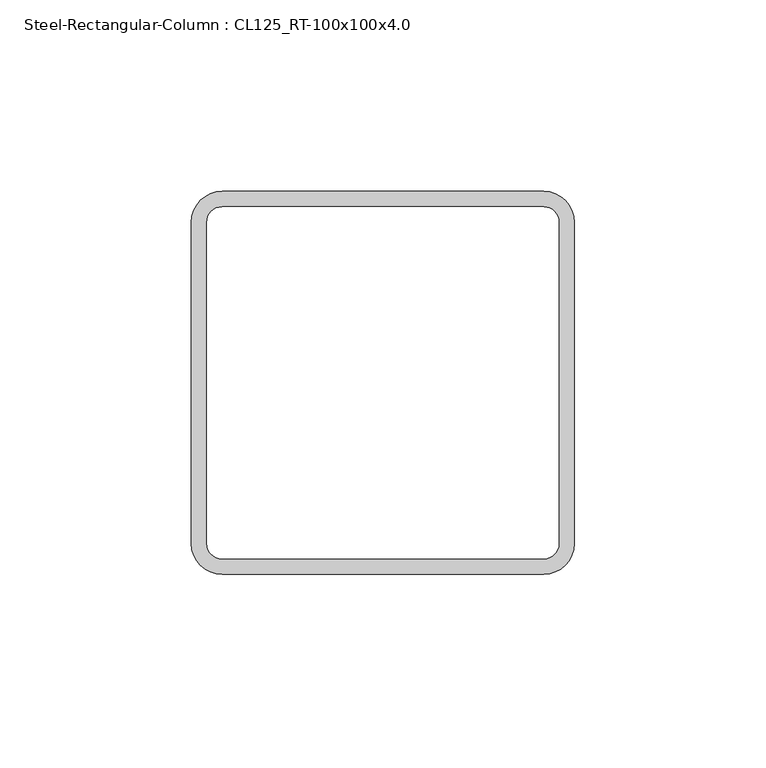
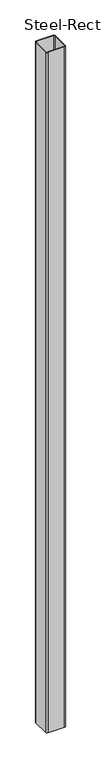
# IFC4 building model written with IfcOpenShell, lengths in millimetres: column geometry, Steel-Rectangular-Column : CL125_RT-100x100x4.0.
# Revit data of these elements (continued)
# Project information (continued)
#     -cfd758078946\" /><element revit_id=\"af7cfdda-f71a-4a09-bb03-63e0c16d5d93-001530cf\" ism_id=\"46a5ded9-4fed-43a0-a06e-bb0fce603002\" /><element revit_id=\"af7cfdda-f71a-4a09-bb03-63e0c16d5d93-001530d1\" ism_id=\"62d05a0c-55f2-4c29-a355-b77f91c84c50\" /><element revit_id=\"af7cfdda-f71a-4a09-bb03-63e0c16d5d93-001530d3\" ism_id=\"eac0c420-7041-45a3-ad98-0cab4f5d8155\" /><element revit_id=\"af7cfdda-f71a-4a09-bb03-63e0c16d5d93-001530d5\" ism_id=\"9f5beb51-429a-4c7b-aa2e-ad2efe601ed6\" /><element revit_id=\"af7cfdda-f71a-4a09-bb03-63e0c16d5d93-001530d7\" ism_id=\"4613af3e-a189-4781-a937-106d789655c9\" /><element revit_id=\"af7cfdda-f71a-4a09-bb03-63e0c16d5d93-001530d9\" ism_id=\"71402e21-51c1-43b7-b8cc-75d2aba247eb\" /><element revit_id=\"af7cfdda-f71a-4a09-bb03-63e0c16d5d93-001530db\" ism_id=\"89101b83-9b84-4f11-b026-90cd564a3900\" /><element revit_id=\"af7cfdda-f71a-4a09-bb03-63e0c16d5d93-001530dd\" ism_id=\"37670781-ce23-4ce1-992b-7a400613c37b\" /><element revit_id=\"af7cfdda-f71a-4a09-bb03-63e0c16d5d93-001530df\" ism_id=\"2316856d-18eb-466b-8ab8-114816378db0\" /><element revit_id=\"af7cfdda-f71a-4a09-bb03-63e0c16d5d93-001530e2\" ism_id=\"da4f1597-5b5a-43a6-aa94-e478ffd6cfc7\" /><element revit_id=\"af7cfdda-f71a-4a09-bb03-63e0c16d5d93-001530e5\" ism_id=\"60805764-efb2-4434-8d81-aed3c3ed3c1b\" /><element revit_id=\"af7cfdda-f71a-4a09-bb03-63e0c16d5d93-001530e8\" ism_id=\"34e34ebb-6481-4bfb-b3d0-cb52295ff652\" /><element revit_id=\"af7cfdda-f71a-4a09-bb03-63e0c16d5d93-001530eb\" ism_id=\"dd5c4d73-1406-4c40-a955-5f9c52d01161\" /><element revit_id=\"af7cfdda-f71a-4a09-bb03-63e0c16d5d93-001530ed\" ism_id=\"cf8abc6b-638f-4bd5-8b66-615be032e220\" /><element revit_id=\"af7cfdda-f71a-4a09-bb03-63e0c16d5d93-001530f0\" ism_id=\"56ce8857-0c24-48d5-82f2-459e263998e2\" /><element revit_id=\"af7cfdda-f71a-4a09-bb03-63e0c16d5d93-001530f2\" ism_id=\"a1f000e8-ea08-442b-8a96-da7657653fd5\" /><element revit_id=\"af7cfdda-f71a-4a09-bb03-63e0c16d5d93-001530f4\" ism_id=\"2625e954-f7fb-41eb-b9bd-1b615ef945fc\" /><element revit_id=\"af7cfdda-f71a-4a09-bb03-63e0c16d5d93-001530f6\" ism_id=\"48469362-393c-4deb-bbb2-ad00180a23fb\" /><element revit_id=\"af7cfdda-f71a-4a09-bb03-63e0c16d5d93-001530f8\" ism_id=\"8e650f6f-0906-45a9-8fb8-35680155d6db\" /><element revit_id=\"af7cfdda-f71a-4a09-bb03-63e0c16d5d93-001530fb\" ism_id=\"f84acaf6-20a1-4df6-afed-1dc07fd0b2e9\" /><element revit_id=\"af7cfdda-f71a-4a09-bb03-63e0c16d5d93-001530fe\" ism_id=\"72816c7e-9128-47f4-b46a-ee567a2a03d6\" /><element revit_id=\"af7cfdda-f71a-4a09-bb03-63e0c16d5d93-00153100\" ism_id=\"c95ab0f8-b4bf-4b7c-bd1d-0423c8ac725a\" /><element revit_id=\"af7cfdda-f71a-4a09-bb03-63e0c16d5d93-00153102\" ism_id=\"32fd4119-6673-4973-aef2-b39ef90310e5\" /><element revit_id=\"af7cfdda-f71a-4a09-bb03-63e0c16d5d93-00153104\" ism_id=\"fd2aa4a6-d123-4100-85b9-db27c20cf6bc\" /><element revit_id=\"af7cfdda-f71a-4a09-bb03-63e0c16d5d93-00153106\" ism_id=\"e00fdefa-e77c-4406-9dbe-3c9122259821\" /><element revit_id=\"af7cfdda-f71a-4a09-bb03-63e0c16d5d93-00153108\" ism_id=\"25e5b79e-07c2-4ffa-a7a9-bf039dd2ad78\" /><element revit_id=\"af7cfdda-f71a-4a09-bb03-63e0c16d5d93-0015310b\" ism_id=\"720021d4-ca74-47c0-9c64-7d0854fa39f5\" /><element revit_id=\"af7cfdda-f71a-4a09-bb03-63e0c16d5d93-0015310d\" ism_id=\"ea922120-0cff-4f8d-a5c2-2841c031873e\" /><element revit_id=\"af7cfdda-f71a-4a09-bb03-63e0c16d5d93-0015310f\" ism_id=\"9d07ca73-3a65-44fe-ab61-476d8d1352d1\" /><element revit_id=\"af7cfdda-f71a-4a09-bb03-63e0c16d5d93-00153111\" ism_id=\"68a2fb30-d213-40c7-a166-dad5a20bd269\" /><element revit_id=\"af7cfdda-f71a-4a09-bb03-63e0c16d5d93-00153113\" ism_id=\"06119775-28f9-44f0-a265-5c57029016d1\" /><element revit_id=\"af7cfdda-f71a-4a09-bb03-63e0c16d5d93-00153115\" ism_id=\"ca133383-8253-4d07-aa92-f507fbb2ee47\" /><element revit_id=\"af7cfdda-f71a-4a09-bb03-63e0c16d5d93-00153117\" ism_id=\"6f4a7c07-4bd3-4c99-b1e4-110c964ccc07\" /><element revit_id=\"af7cfdda-f71a-4a09-bb03-63e0c16d5d93-00153119\" ism_id=\"ee1f865b-98a9-4ff1-a84c-52926e8f3566\" /><element revit_id=\"af7cfdda-f71a-4a09-bb03-63e0c16d5d93-0015311b\" ism_id=\"4fd7bd5c-7c46-4e79-a72b-dab4a1d98f33\" /><element revit_id=\"af7cfdda-f71a-4a09-bb03-63e0c16d5d93-0015311e\" ism_id=\"9ca0cac6-aaff-412a-b9c1-a8be985bc44a\" /><element revit_id=\"af7cfdda-f71a-4a09-bb03-63e0c16d5d93-00153121\" ism_id=\"73123639-76b5-46f0-a49e-b26af36d93b1\" /><element revit_id=\"af7cfdda-f71a-4a09-bb03-63e0c16d5d93-00153123\" ism_id=\"f74e8cb9-a93d-4aaa-985b-c0ed9befad19\" /><element revit_id=\"af7cfdda-f71a-4a09-bb03-63e0c16d5d93-00153126\" ism_id=\"5778daa1-b4cb-4cc3-9b7d-323562a47fba\" /><element revit_id=\"af7cfdda-f71a-4a09-bb03-63e0c16d5d93-00153129\" ism_id=\"2d7457d2-8978-4c95-9056-ebbaed3263eb\" /><element revit_id=\"af7cfdda-f71a-4a09-bb03-63e0c16d5d93-0015312c\" ism_id=\"48b420ce-6767-430a-aadc-695c25361a2d\" /><element revit_id=\"af7cfdda-f71a-4a09-bb03-63e0c16d5d93-0015312e\" ism_id=\"fc34038c-136d-4d55-b951-9cc35899fd33\" /><element revit_id=\"af7cfdda-f71a-4a09-bb03-63e0c16d5d93-00153130\" ism_id=\"e7a25938-3b91-4519-a48d-86fdd79489d5\" /><element revit_id=\"af7cfdda-f71a-4a09-bb03-63e0c16d5d93-00153133\" ism_id=\"c81dfd8c-579c-4d77-ab89-bf1f415d9cc6\" /><element revit_id=\"af7cfdda-f71a-4a09-bb03-63e0c16d5d93-00153136\" ism_id=\"5756a4b4-84ca-418c-b9f6-2d2370afca2f\" /><element revit_id=\"af7cfdda-f71a-4a09-bb03-63e0c16d5d93-0015313a\" ism_id=\"09a9cede-a757-4d8e-a722-6140af98bc61\" /><element revit_id=\"af7cfdda-f71a-4a09-bb03-63e0c16d5d93-0015313d\" ism_id=\"ac9b583c-7f63-4351-8b69-3967279b234c\" /><element revit_id=\"af7cfdda-f71a-4a09-bb03-63e0c16d5d93-00153140\" ism_id=\"1a52584d-6b21-4de6-bb42-5b9bdd6f24e9\" /><element revit_id=\"af7cfdda-f71a-4a09-bb03-63e0c16d5d93-00153143\" ism_id=\"6c2e2bc0-8432-4c98-9292-cbb2182bd4b0\" /><element revit_id=\"af7cfdda-f71a-4a09-bb03-63e0c16d5d93-00153145\" ism_id=\"644bb900-7654-42c5-a9b7-996a2197f6d0\" /><element revit_id=\"af7cfdda-f71a-4a09-bb03-63e0c16d5d93-00153148\" ism_id=\"a1bca0bd-75db-464c-b27a-2a69d9b4ad3d\" /><element revit_id=\"af7cfdda-f71a-4a09-bb03-63e0c16d5d93-0015314a\" ism_id=\"ea29955b-34f2-409a-aefa-e6adfe75349e\" /><element revit_id=\"af7cfdda-f71a-4a09-bb03-63e0c16d5d93-0015314d\" ism_id=\"800fef33-e5e1-422c-b708-e9394bbeefcc\" /><element revit_id=\"af7cfdda-f71a-4a09-bb03-63e0c16d5d93-0015314f\" ism_id=\"86259dca-8773-4253-ac56-e71252267c8a\" /><element revit_id=\"af7cfdda-f71a-4a09-bb03-63e0c16d5d93-00153152\" ism_id=\"d15a0ad2-db9f-420d-bea3-41a78a0eb330\" /><element revit_id=\"af7cfdda-f71a-4a09-bb03-63e0c16d5d93-00153155\" ism_id=\"bd27f420-df49-4abe-bd96-8e48e7f4efcb\" /><element revit_id=\"af7cfdda-f71a-4a09-bb03-63e0c16d5d93-00153157\" ism_id=\"5d451f94-860d-4cc3-a4fa-51a9f3126e33\" /><element revit_id=\"af7cfdda-f71a-4a09-bb03-63e0c16d5d93-0015315a\" ism_id=\"4234158a-994a-492b-85da-6108709b7232\" /><element revit_id=\"af7cfdda-f71a-4a09-bb03-63e0c16d5d93-0015315c\" ism_id=\"ca24c92d-986b-417f-812f-024ab15e24c8\" /><element revit_id=\"af7cfdda-f71a-4a09-bb03-63e0c16d5d93-0015315f\" ism_id=\"699ec3b0-0151-4110-b054-14418651f324\" /><element revit_id=\"af7cfdda-f71a-4a09-bb03-63e0c16d5d93-00153161\" ism_id=\"38ecdeac-3d85-48dd-82c1-53fe93f49beb\" /><element revit_id=\"af7cfdda-f71a-4a09-bb03-63e0c16d5d93-00153163\" ism_id=\"1340aefd-b79c-4264-8a49-d0a0504eff8c\" /><element revit_id=\"af7cfdda-f71a-4a09-bb03-63e0c16d5d93-00153165\" ism_id=\"1b6167c2-fb26-4b8d-916b-d835d89896e7\" /><element revit_id=\"af7cfdda-f71a-4a09-bb03-63e0c16d5d93-00153167\" ism_id=\"290d3d83-57eb-4125-aecb-a977a5fcf5ca\" /><element revit_id=\"af7cfdda-f71a-4a09-bb03-63e0c16d5d93-00153169\" ism_id=\"105c9b97-1c70-4237-82ac-8404a3e8e6a6\" /><element revit_id=\"af7cfdda-f71a-4a09-bb03-63e0c16d5d93-0015316c\" ism_id=\"1726c5bb-05e2-4959-9da2-4227f0219f00\" /><element revit_id=\"af7cfdda-f71a-4a09-bb03-63e0c16d5d93-0015316e\" ism_id=\"d919ee9c-caed-4119-b451-e3644db952c8\" /><element revit_id=\"af7cfdda-f71a-4a09-bb03-63e0c16d5d93-00153170\" ism_id=\"1b1fab26-60c4-40ed-b31b-b177eda246ce\" /><element revit_id=\"af7cfdda-f71a-4a09-bb03-63e0c16d5d93-00153172\" ism_id=\"ea9b5221-a1f2-4796-8cca-f7872ab69cbd\" /><element revit_id=\"af7cfdda-f71a-4a09-bb03-63e0c16d5d93-00153174\" ism_id=\"660b40b2-06fb-4b62-b987-28a171e473fe\" /><element revit_id=\"af7cfdda-f71a-4a09-bb03-63e0c16d5d93-00153176\" ism_id=\"767be0d9-c5ba-4ad3-a52d-efd60031fc9a\" /><element revit_id=\"af7cfdda-f71a-4a09-bb03-63e0c16d5d93-00153178\" ism_id=\"6fbe93ce-4ed7-4596-88fc-71dafe48803e\" /><element revit_id=\"af7cfdda-f71a-4a09-bb03-63e0c16d5d93-0015317a\" ism_id=\"27d7b093-4eb7-47aa-b123-5388a6327d7f\" /><element revit_id=\"af7cfdda-f71a-4a09-bb03-63e0c16d5d93-0015317c\" ism_id=\"9073a947-5952-42fe-b37a-cdfed3ca30c7\" /><element revit_id=\"af7cfdda-f71a-4a09-bb03-63e0c16d5d93-0015317e\" ism_id=\"1888f060-aa3c-4494-8f30-a80ca2311216\" /><element revit_id=\"af7cfdda-f71a-4a09-bb03-63e0c16d5d93-00153181\" ism_id=\"c0491dc2-5df2-4c14-b988-e117f6f511a2\" /><element revit_id=\"af7cfdda-f71a-4a09-bb03-63e0c16d5d93-00153184\" ism_id=\"4f44b9aa-c092-46fe-bf9b-2d1be872d419\" /><element revit_id=\"af7cfdda-f71a-4a09-bb03-63e0c16d5d93-00153186\" ism_id=\"eb560801-76cf-40a8-a181-31cd32aca14f\" /><element revit_id=\"af7cfdda-f71a-4a09-bb03-63e0c16d5d93-00153189\" ism_id=\"8d1e5f00-41d5-42c1-9b4f-a8c2eb689a72\" /><element revit_id=\"af7cfdda-f71a-4a09-bb03-63e0c16d5d93-0015318b\" ism_id=\"caf6c2dc-0e9e-46a9-a3e1-71316081ff61\" /><element revit_id=\"af7cfdda-f71a-4a09-bb03-63e0c16d5d93-0015318d\" ism_id=\"4d149f88-f5b9-4943-8765-090324e0a65d\" /><element revit_id=\"af7cfdda-f71a-4a09-bb03-63e0c16d5d93-0015318f\" ism_id=\"75865cf2-3adc-4a52-a778-fc6fb65fcdcb\" /><element revit_id=\"af7cfdda-f71a-4a09-bb03-63e0c16d5d93-00153191\" ism_id=\"f9320017-2083-48f1-8aff-e6ba958fb1c5\" /><element revit_id=\"af7cfdda-f71a-4a09-bb03-63e0c16d5d93-00153193\" ism_id=\"38a61c12-98f2-47b1-843d-8351040e24d2\" /><element revit_id=\"af7cfdda-f71a-4a09-bb03-63e0c16d5d93-00153196\" ism_id=\"af709a9c-b664-480b-be0d-fb01aac630f2\" /><element revit_id=\"af7cfdda-f71a-4a09-bb03-63e0c16d5d93-00153199\" ism_id=\"a4c2867c-ca2a-4112-b86c-4e6563e3dc63\" /><element revit_id=\"14a48413-84c4-4e00-9e64-4f618415469a-0013ce74\" ism_id=\"F2ADF140-E21A-4820-8170-6F63D956DCAD\" /><element revit_id=\"14a48413-84c4-4e00-9e64-4f618415469a-0013ce74\" ism_id=\"B35A310E-4F33-462b-819C-3ADD300C0CEB\" /><element revit_id=\"14a48413-84c4-4e00-9e64-4f618415469a-0013ce74\" ism_id=\"711054EC-0DB2-46e3-AD20-004560300C00\" /><element revit_id=\"14a48413-84c4-4e00-9e64-4f618415469a-0013ce6e\" ism_id=\"B5C54EC9-8EBD-4860-AB72-EF5791AED394\" /><element revit_id=\"14a48413-84c4-4e00-9e64-4f618415469a-0013e793\" ism_id=\"0A7B8D02-9EA4-4aa9-A41A-E30BB5B6B6C5\" /><element revit_id=\"14a48413-84c4-4e00-9e64-4f618415469a-0013e793\" ism_id=\"714BBD27-DB58-47da-B54C-5806291C2D3C\" /><element revit_id=\"14a48413-84c4-4e00-9e64-4f618415469a-0013e793\" ism_id=\"F36E62C1-13EE-4807-A3C1-899E23E0BEDE\" /><element revit_id=\"14a48413-84c4-4e00-9e64-4f618415469a-0013e793\" ism_id=\"F5448801-679E-44d6-8F46-E676344F8165\" /><element revit_id=\"14a48413-84c4-4e00-9e64-4f618415469a-0013e793\" ism_id=\"846DCB0C-E06B-4978-9D43-E1CC0FDE7595\" /><element revit_id=\"14a48413-84c4-4e00-9e64-4f618415469a-0013e793\" ism_id=\"2ADF82B8-986D-4f44-85DE-89D921292160\" /><element revit_id=\"14a48413-84c4-4e00-9e64-4f618415469a-0013e793\" ism_id=\"7AF371ED-051B-4a30-8826-11F11C212B73\" /><element revit_id=\"14a48413-84c4-4e00-9e64-4f618415469a-0013e793\" ism_id=\"2FE74006-ADDA-412f-A522-853919E62B4D\" /><element revit_id=\"14a48413-84c4-4e00-9e64-4f618415469a-0013e793\" ism_id=\"09B63641-D581-4a6c-A18E-54C17EC989A4\" /><element revit_id=\"14a48413-84c4-4e00-9e64-4f618415469a-0013e793\" ism_id=\"0DD6B52A-77D0-45a1-82B1-8236ED57078C\" /><element revit_id=\"14a48413-84c4-4e00-9e64-4f618415469a-0013e793\" ism_id=\"35D311D2-DEB8-4469-97DE-110B6DF5B84D\" /><element revit_id=\"14a48413-84c4-4e00-9e64-4f618415469a-0013e79
#     3\" ism_id=\"0D3CCDE5-CFF9-431b-A4BD-01BF6636D6BD\" /><element revit_id=\"14a48413-84c4-4e00-9e64-4f618415469a-0013e793\" ism_id=\"C62B2A5B-024A-47ac-B030-C17A67E64A7B\" /><element revit_id=\"14a48413-84c4-4e00-9e64-4f618415469a-0013e793\" ism_id=\"944C6E43-E607-48c3-8358-9E6CB88346E7\" /><element revit_id=\"14a48413-84c4-4e00-9e64-4f618415469a-0013e793\" ism_id=\"A4B1F42D-B1C2-4ad2-8AD6-DB0D5E05998D\" /><element revit_id=\"14a48413-84c4-4e00-9e64-4f618415469a-0013e793\" ism_id=\"007E6C70-1139-4b48-B003-C76FAD4C249A\" /><element revit_id=\"14a48413-84c4-4e00-9e64-4f618415469a-0013e793\" ism_id=\"9941AC94-F03A-464c-9912-04590E0C31E0\" /><element revit_id=\"14a48413-84c4-4e00-9e64-4f618415469a-0013e793\" ism_id=\"CFD98B8D-8FF4-4e71-A909-0FE7DBCE924E\" /><element revit_id=\"14a48413-84c4-4e00-9e64-4f618415469a-0013e793\" ism_id=\"58262161-98E6-45c8-B2BD-4508105FF662\" /><element revit_id=\"14a48413-84c4-4e00-9e64-4f618415469a-0013e793\" ism_id=\"66AB4841-610A-4883-97F7-1282A56484E1\" /><element revit_id=\"14a48413-84c4-4e00-9e64-4f618415469a-0013e793\" ism_id=\"D2B324BE-BBD6-49da-9730-60EA7AD4D3A0\" /><element revit_id=\"14a48413-84c4-4e00-9e64-4f618415469a-0013e793\" ism_id=\"92A8ECE7-C053-46b1-92ED-F2C041617E7B\" /><element revit_id=\"14a48413-84c4-4e00-9e64-4f618415469a-0013e793\" ism_id=\"B4C4BDB0-65C4-4016-9C78-DBD77E229523\" /><element revit_id=\"14a48413-84c4-4e00-9e64-4f618415469a-0013e793\" ism_id=\"57270646-162F-4c83-BDB7-A5FBEA9120BD\" /><element revit_id=\"14a48413-84c4-4e00-9e64-4f618415469a-0013e793\" ism_id=\"BDEF733F-00AA-4eee-B6C6-50229FC1D236\" /><element revit_id=\"14a48413-84c4-4e00-9e64-4f618415469a-0013e793\" ism_id=\"84A94E1E-3074-40f4-9690-97191755F019\" /><element revit_id=\"14a48413-84c4-4e00-9e64-4f618415469a-0013e793\" ism_id=\"8A7D913D-7967-4718-912D-B83DF0AD2EDD\" /><element revit_id=\"14a48413-84c4-4e00-9e64-4f618415469a-0013e793\" ism_id=\"83553D70-90FA-469c-B5C3-EF03F3FC6475\" /><element revit_id=\"14a48413-84c4-4e00-9e64-4f618415469a-0013e793\" ism_id=\"6880C1E4-C50B-4c1b-B61C-23F2D8C46873\" /><element revit_id=\"14a48413-84c4-4e00-9e64-4f618415469a-0013e793\" ism_id=\"08594C43-CD40-47de-A3BA-8BFB47F64994\" /><element revit_id=\"14a48413-84c4-4e00-9e64-4f618415469a-0013e793\" ism_id=\"7D2E11FA-A5E1-4434-B9BE-AABA1A16CA03\" /><element revit_id=\"14a48413-84c4-4e00-9e64-4f618415469a-0013e793\" ism_id=\"D892DFA4-5441-4ad2-A390-253492293B1B\" /><element revit_id=\"14a48413-84c4-4e00-9e64-4f618415469a-0013e793\" ism_id=\"E5A32FE6-89C4-49f1-B3B9-1CABE7C48A4D\" /><element revit_id=\"14a48413-84c4-4e00-9e64-4f618415469a-0013e793\" ism_id=\"8AE872C2-5DBE-47c5-934B-7E964A84B589\" /><element revit_id=\"14a48413-84c4-4e00-9e64-4f618415469a-0013e793\" ism_id=\"3C847B60-488A-4604-A400-16A3A65E919B\" /><element revit_id=\"14a48413-84c4-4e00-9e64-4f618415469a-0013e793\" ism_id=\"DBEC432A-3F7B-4266-AD99-2A937DC70BCF\" /><element revit_id=\"14a48413-84c4-4e00-9e64-4f618415469a-0013e793\" ism_id=\"59403DD6-7A51-48aa-A3BE-962457E6F10E\" /><element revit_id=\"14a48413-84c4-4e00-9e64-4f618415469a-0013e793\" ism_id=\"11CDDF5D-38B6-43b2-A291-FC188BE232BC\" /><element revit_id=\"14a48413-84c4-4e00-9e64-4f618415469a-0013e793\" ism_id=\"10BF2843-EFC9-4136-933C-5B270D970277\" /><element revit_id=\"14a48413-84c4-4e00-9e64-4f618415469a-0013e793\" ism_id=\"E1B09A9C-F6C6-47d9-976B-E313C0E3F52B\" /><element revit_id=\"14a48413-84c4-4e00-9e64-4f618415469a-0013e793\" ism_id=\"A3A22EC3-26C8-4588-A0AB-AFAE02DF267E\" /><element revit_id=\"14a48413-84c4-4e00-9e64-4f618415469a-0013e793\" ism_id=\"114828FC-BDC1-4343-9119-BCB5395DAA64\" /><element revit_id=\"14a48413-84c4-4e00-9e64-4f618415469a-0013e793\" ism_id=\"797626F9-3558-4623-826F-15FB93088CB3\" /><element revit_id=\"14a48413-84c4-4e00-9e64-4f618415469a-0013e793\" ism_id=\"4BF369CD-DF09-4346-96CB-C6C6380A2599\" /><element revit_id=\"14a48413-84c4-4e00-9e64-4f618415469a-0013e793\" ism_id=\"722B46BA-61C4-44a1-9ECF-325B60B6688D\" /><element revit_id=\"14a48413-84c4-4e00-9e64-4f618415469a-0013e793\" ism_id=\"C33DBE84-19C1-4379-AB6E-A41F7420F18C\" /><element revit_id=\"14a48413-84c4-4e00-9e64-4f618415469a-0013e793\" ism_id=\"1F2D3B75-66F2-4d88-A1DD-647969477B86\" /><element revit_id=\"14a48413-84c4-4e00-9e64-4f618415469a-0013e793\" ism_id=\"DFBF96B2-410A-4f39-80C4-D8CF78561C93\" /><element revit_id=\"14a48413-84c4-4e00-9e64-4f618415469a-0013e793\" ism_id=\"D6793CD3-AB64-417c-9C28-8B18A0A2D336\" /><element revit_id=\"14a48413-84c4-4e00-9e64-4f618415469a-0013e793\" ism_id=\"90884AC0-EA00-4caa-86E1-E6B886FD90ED\" /><element revit_id=\"14a48413-84c4-4e00-9e64-4f618415469a-0013e793\" ism_id=\"64BC7B89-F7C8-4dae-A5C8-F10DF9E5F6BA\" /><element revit_id=\"14a48413-84c4-4e00-9e64-4f618415469a-0013e793\" ism_id=\"D82E4D85-2728-40e5-9F60-1C7FB2990D78\" /><element revit_id=\"14a48413-84c4-4e00-9e64-4f618415469a-0013e793\" ism_id=\"1E6D05B9-BF84-4669-AA27-948ADA1D511E\" /><element revit_id=\"14a48413-84c4-4e00-9e64-4f618415469a-0013e793\" ism_id=\"73608CB2-EB94-466e-883D-814030EF49D6\" /><element revit_id=\"14a48413-84c4-4e00-9e64-4f618415469a-0013e793\" ism_id=\"4EAF07EF-4E08-4065-9F08-BF69D4413867\" /><element revit_id=\"14a48413-84c4-4e00-9e64-4f618415469a-0013e0e9\" ism_id=\"05D74241-6318-4cac-95F5-7B878260D5B5\" /></element_binding><reinforcement_properties /><operation_settings><coordinate_mapping x=\"0\" y=\"0\" z=\"0\" /></operation_settings></ism>"
#   Building Name = "FIRE WATER PUMP BUILDING"
#   Project Status = "Project Status"
#   Client Name = "현대엔지니어링"
#   Project Address = "서울시 종로구 율곡로 75(계동)"
#   Project Name = "TAKHIATASH POWER PLANT EFFICIENCY IMPROVEMENT PROJECT / 우즈베키스탄"
#   Project Number = "BEUZ1602"
#   F01) Building Name = "FIRE WATER PUMP BUILDING"
#   F11) Project Building Tag_Type-1 = "BI aWBS"
#   F12) Project Building Tag_Type-2 = "BI aWBS"
#   F13) Project Facility Code = "621"
#   F21) Structural Type = "STEEL"
#   F31) Standard Building Code = "E204"
#   F41) Discipline = "Architecture"
#   F51) Plan Start Date-Engineering = "2018-01-01"
#   F52) Plan Finish Date-Engineering = "2018-09-13"
#   F53) Duration = "255"
#   F61) Plan Start Date-Construction = "2018-09-14"
#   F62) Plan Finish Date-Construction = "2019-12-02"
#   F63) Duration = "444"
#   F91) Plant Type = "2GTG+2STG+1HRSG"
#   F92) KKS Structures, Building = "UAB"
#   P01) Project Name = "TAKHIATASH POWER PLANT EFFICIENCY IMPROVEMENT PROJECT / 우즈베키스탄"
#   P02) Project Configuration = "2 GTG + 2 HRSG + 2STG, 2 x 250MW"
#   P03) Project Abbreviation = "UTCC"
#   P04) Project Code = "BEUZ1602"
#   P05) Project Stage = "실행"
#   P06) Project Location = "Takhiatash / Uzbekistan"
#   P07) Project Owner = "우즈베키스탄 전력청"
#   P08) Project O.E = "GAS Natural Fenosa"
#   P09) Project Schedule = "2017.10.01 ~ 2020.08.08"
#   P10) Basic Wind Speed = "48m/sec_ASCE7-05"
#   P11) Seismic = "SDS_0.15_ASCE7-05"
#   P12) Soil = "SD_ASCE7-05"
#   P13) Soil Capacity = "400 kN/m2_Soil Replacement"
#   P14) Pile Capacity = "1000 kN_D600 Board Pile"
# Type "Steel-Rectangular-Column : CL125_RT-100x100x4.0"
#   Surface Area = 0.386 m²/m
#   b = 100 mm
#   h = 100 mm
#   tr = 8 mm
#   t = 4 mm
#   Section Area = 14.95 cm²
#   Mass per Unit Length = 11.70 kg/m
#   hec_material4 [instance default] = none
#   hec_material3 [instance default] = none
#   hec_material2 [instance default] = none
#   hec_material1 [instance default] = none
#   Structural Material [instance default] = Steel, 45-345
# Element 1 (IfcColumn, "Steel-Rectangular-Column : CL125_RT-100x100x4.0")
#   Structural Material = S01AA007-00001_Main Steel Structure Fabrication Work_Shelter/Building_Girth & Purlin
#   Materials on its faces: "S01AA007-00001_Main Steel Structure Fabrication Work_Shelter/Building_Girth & Purlin"
# Materials
#   "Steel, 45-345": class "Metal", colour RGB 189 187 185, transparency 0, Description = "Steel 345 MPa", Cost = 0
#   "S01AA007-00001_Main Steel Structure Fabrication Work_Shelter/Building_Girth & Purlin": class "Metal", colour RGB 120 120 120, transparency 0, Comments = "(30KG/M>Weight)", Description = "Structural steel 50ksi", W00) Work Master Code = "S01AA007-00001", W01) Work Master_Lv1 = "Main Steel Structure Fabrication Work", W02) Work Master_Lv2 = "Shelter/Building", W03) Work Master_Spec.1 = "Girth & Purlin", Cost = 0
